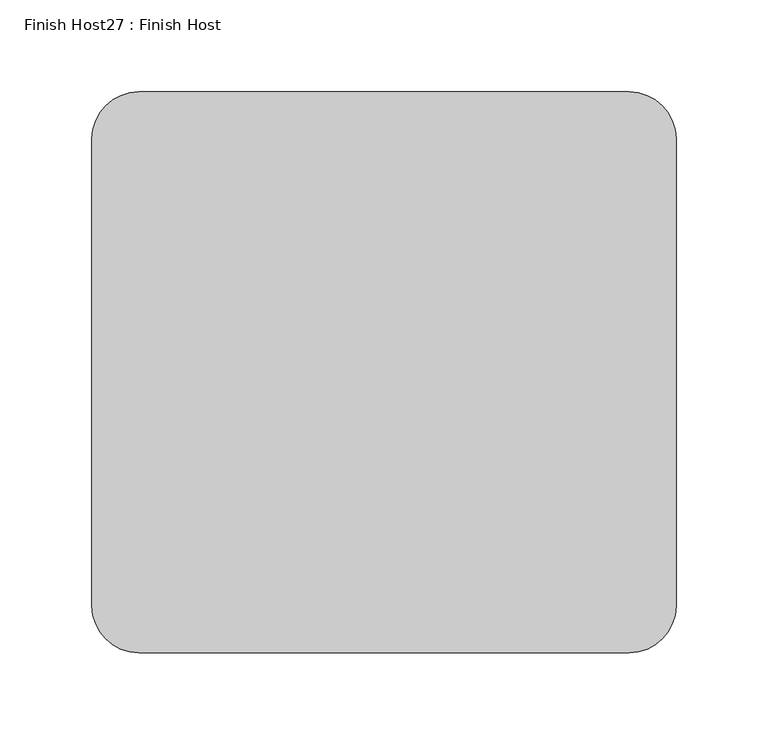
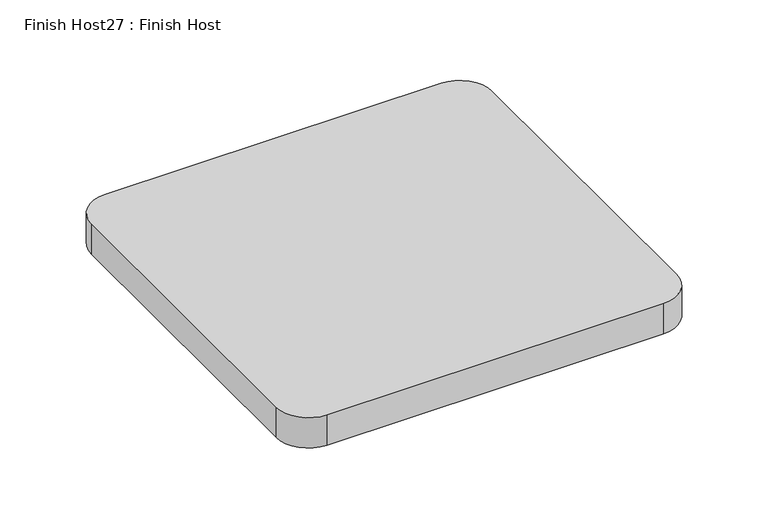
"""IFC4 building model written with IfcOpenShell, lengths in millimetres: proxy geometry, Finish Host27 : Finish Host."""

from ifc_helpers import new_model, si_unit, point, frame_2d, origin, origin_with_axes, place, context, project, spatial, polyline, circle_curve, trimmed, segment, composite_curve, outline, extrude, source, transform, mapped, element, save


def finish_host27_finish_host_bffc5e38(model_context):
    return source(origin(), model_context, "Body", "SweptSolid", [
        extrude(outline(composite_curve([segment(polyline([(-14128.7939795, 11089.4419385), (-14128.7939795, 11343.4419385)]), True, "CONTINUOUS"), segment(trimmed(circle_curve(frame_2d((-14103.3939795, 11343.4419385)), 25.4), [point((-14128.7939795, 11343.4419385))], [point((-14103.3939795, 11368.8419385))], False, "CARTESIAN"), True, "CONTINUOUS"), segment(polyline([(-14103.3939795, 11368.8419385), (-13836.6939795, 11368.8419385)]), True, "CONTINUOUS"), segment(trimmed(circle_curve(frame_2d((-13836.6939795, 11343.4419385)), 25.4), [point((-13836.6939795, 11368.8419385))], [point((-13811.2939795, 11343.4419385))], False, "CARTESIAN"), True, "CONTINUOUS"), segment(polyline([(-13811.2939795, 11343.4419385), (-13811.2939795, 11089.4419385)]), True, "CONTINUOUS"), segment(trimmed(circle_curve(frame_2d((-13836.6939795, 11089.4419385)), 25.4), [point((-13811.2939795, 11089.4419385))], [point((-13836.6939795, 11064.0419385))], False, "CARTESIAN"), True, "CONTINUOUS"), segment(polyline([(-13836.6939795, 11064.0419385), (-14103.3939795, 11064.0419385)]), True, "CONTINUOUS"), segment(trimmed(circle_curve(frame_2d((-14103.3939795, 11089.4419385)), 25.4), [point((-14103.3939795, 11064.0419385))], [point((-14128.7939795, 11089.4419385))], False, "CARTESIAN"), True, "CONTINUOUS")], self_intersect=False)), origin_with_axes(), (0.0, 0.0, 1.0), 25.4),
    ])


if __name__ == "__main__":
    model = new_model("IFC4")
    model_context = context("Model", 3, world=origin())
    ifc_project = project(units=[si_unit("LENGTHUNIT", "METRE", prefix="MILLI")], contexts=[model_context])
    site = spatial("IfcSite", under=ifc_project)
    building = spatial("IfcBuilding", under=site)
    placement = place(None, origin())
    finish_host27_finish_host_shape = finish_host27_finish_host_bffc5e38(model_context)
    element("IfcBuildingElementProxy", 1, Name="Finish Host27 : Finish Host", ObjectType="Finish Host27 : Finish Host", at=placement, inside=building, context=model_context, shape_type="MappedRepresentation", body=[
        mapped(finish_host27_finish_host_shape, transform((0.0, 0.0, 0.0), x_axis=(1.0, 0.0, 0.0), y_axis=(0.0, 1.0, 0.0), z_axis=(0.0, 0.0, 1.0))),
    ])
    save(model, "model.ifc")

# Revit data of these elements
# Type "Finish Host27 : Finish Host"
#   Countertop Material = Fabric - Teknion - S614 - Saturate - Sepia
# Element 1 (IfcBuildingElementProxy, "Finish Host27 : Finish Host")
#   Materials on its faces: "Fabric - Teknion - S614 - Saturate - Sepia"
# Materials
#   "Fabric - Teknion - S614 - Saturate - Sepia": class "Fabric", colour RGB 37 34 32, transparency 0, Model = "S614", Manufacturer = "Teknion Studio", URL = "http://www.teknionstudio.com/", Description = "Sepia Saturate", Cost = 0
